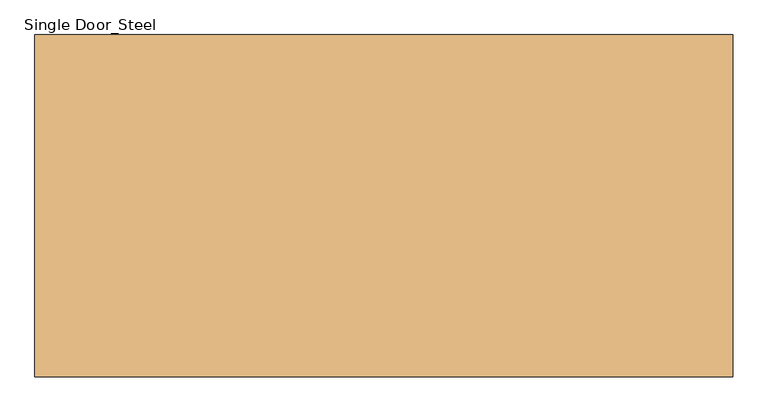
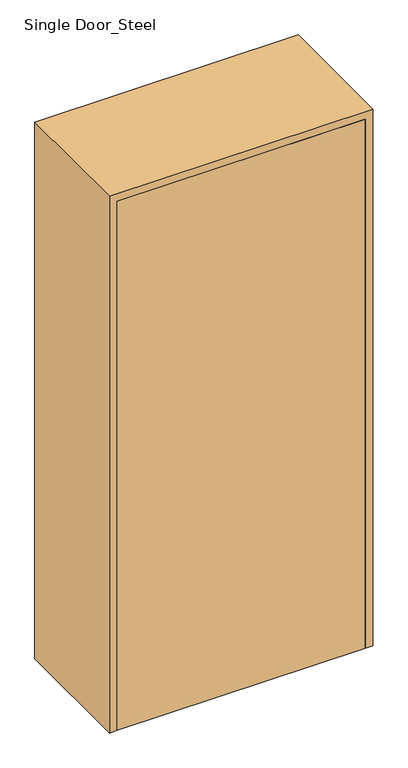
"""IFC4 building model written with IfcOpenShell, lengths in millimetres: door geometry, Single Door_Steel : H_DR_AMB_Single Door_Steel_W1000xH2150."""

from ifc_helpers import new_model, si_unit, origin, origin_with_axes, place, context, project, spatial, polyline, outline, extrude, faceted_brep, source, transform, mapped, element, save


def single_door_steel_cad2a4f8(model_context):
    return source(origin(), model_context, "Body", "SolidModel", [
        extrude(outline(polyline([(470.0, -245.0), (-470.0, -245.0), (-470.0, -210.0), (470.0, -210.0), (470.0, -245.0)])), origin_with_axes(), (0.0, 0.0, 1.0), 2120.0),
        faceted_brep([(470.0, -245.0, 0.0), (470.0, -210.0, 0.0), (450.0, -210.0, 0.0), (450.0, 210.0, 0.0), (470.0, 210.0, 0.0), (470.0, 245.0, 0.0), (500.0, 245.0, 0.0), (500.0, -245.0, 0.0), (500.0, -245.0, 2150.0), (-500.0, -245.0, 2150.0), (-500.0, -245.0, 0.0), (-470.0, -245.0, 0.0), (-470.0, -245.0, 2120.0), (470.0, -245.0, 2120.0), (500.0, 245.0, 2150.0), (470.0, 245.0, 2120.0), (-470.0, 245.0, 2120.0), (-470.0, 245.0, 0.0), (-500.0, 245.0, 0.0), (-500.0, 245.0, 2150.0), (470.0, 210.0, 2120.0), (450.0, 210.0, 2100.0), (-450.0, 210.0, 2100.0), (-450.0, 210.0, 0.0), (-470.0, 210.0, 0.0), (-470.0, 210.0, 2120.0), (450.0, -210.0, 2100.0), (470.0, -210.0, 2120.0), (-470.0, -210.0, 2120.0), (-470.0, -210.0, 0.0), (-450.0, -210.0, 0.0), (-450.0, -210.0, 2100.0)], [[[0, 1, 2, 3, 4, 5, 6, 7]], [[7, 8, 9, 10, 11, 12, 13, 0]], [[6, 14, 8, 7]], [[5, 15, 16, 17, 18, 19, 14, 6]], [[4, 20, 15, 5]], [[3, 21, 22, 23, 24, 25, 20, 4]], [[2, 26, 21, 3]], [[1, 27, 28, 29, 30, 31, 26, 2]], [[0, 13, 27, 1]], [[12, 11, 29, 28]], [[11, 10, 18, 17, 24, 23, 30, 29]], [[19, 18, 10, 9]], [[25, 24, 17, 16]], [[31, 30, 23, 22]], [[14, 19, 9, 8]], [[20, 25, 16, 15]], [[26, 31, 22, 21]], [[13, 12, 28, 27]]]),
    ])


if __name__ == "__main__":
    model = new_model("IFC4")
    model_context = context("Model", 3, world=origin())
    ifc_project = project(units=[si_unit("LENGTHUNIT", "METRE", prefix="MILLI")], contexts=[model_context])
    site = spatial("IfcSite", under=ifc_project)
    building = spatial("IfcBuilding", under=site)
    placement = place(None, origin())
    single_door_steel_shape = single_door_steel_cad2a4f8(model_context)
    element("IfcDoor", 1, ObjectType="Single Door_Steel : H_DR_AMB_Single Door_Steel_W1000xH2150", at=placement, inside=building, context=model_context, shape_type="MappedRepresentation", body=[
        mapped(single_door_steel_shape, transform((0.0, 0.0, 0.0), x_axis=(1.0, 0.0, 0.0), y_axis=(0.0, 1.0, 0.0), z_axis=(0.0, 0.0, 1.0))),
    ])
    save(model, "model.ifc")

# Revit data of these elements
# Type "Single Door_Steel : H_DR_AMB_Single Door_Steel_W1000xH2150"
#   Type Mark = "364"
#   Analytic Construction = "<None>"
#   프레임 투영 외부. = 25.000 mm
#   프레임 투영 내부. = 25.000 mm
#   프레임 폭 = 75.000 mm
#   Height = 2150.000 mm
#   Width = 1000.000 mm
#   Define Thermal Properties by = 1
#   문 패널 = none
#   문 프레임 = none
#   Function = (empty or 0)
#   Wall Closure = (empty or 0)
